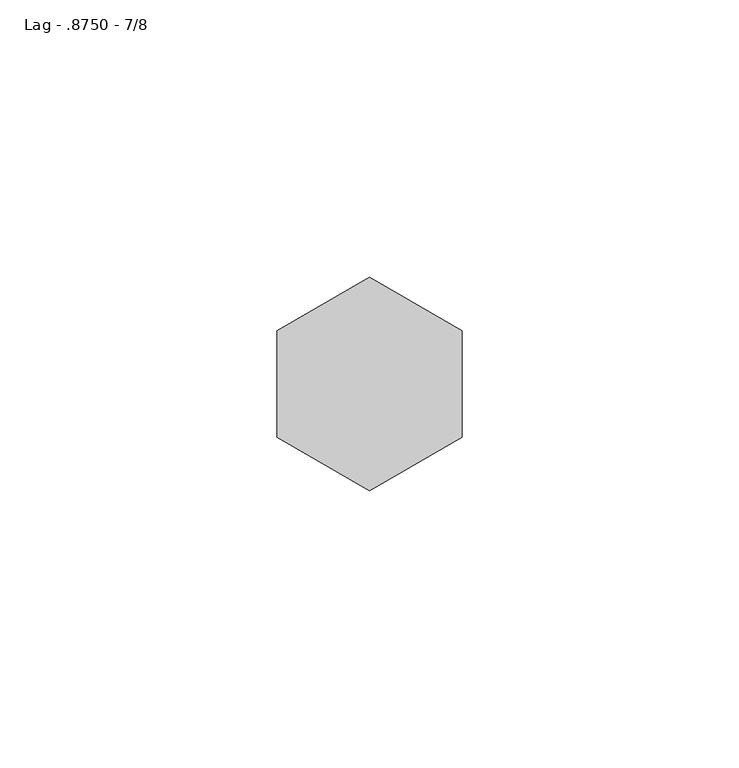
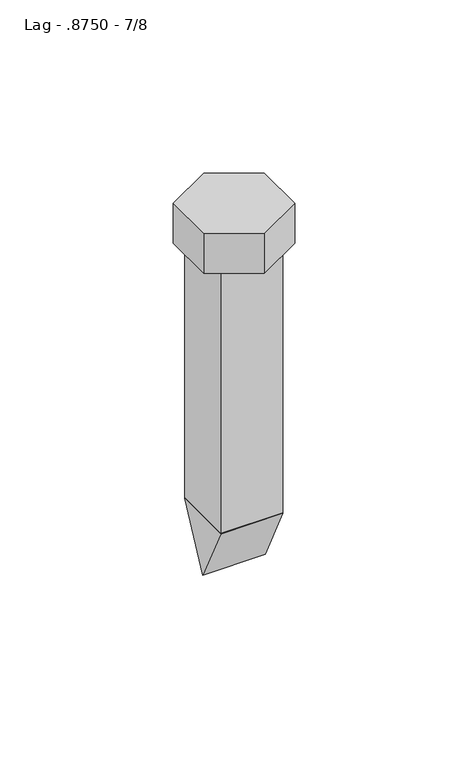
"""IFC4 building model written with IfcOpenShell, lengths in millimetres: fastener geometry, 060523 - W_P_C - Fastenings - Generic - SQUARE : Lag - .8750 - 7/8."""

from ifc_helpers import new_model, si_unit, frame, origin, origin_with_axes, place, context, project, spatial, polyline, outline, extrude, source, transform, mapped, element, save


def lag_8750_7_8_9ca2a517(model_context):
    return source(origin(), model_context, "Body", "SweptSolid", [
        extrude(outline(polyline([(0.0, -124.3210937), (-11.3605469, -101.6), (11.3605469, -101.6), (0.0, -124.3210937)])), frame((-11.3605469, 0.0, 0.0), z_axis=(1.0, 0.0, 0.0), x_axis=(0.0, 1.0, 0.0)), (0.0, 0.0, 1.0), 22.7210938),
        extrude(outline(polyline([(-16.66875, 9.6237073), (0.0, 19.2474146), (16.66875, 9.6237073), (16.66875, -9.6237073), (0.0, -19.2474146), (-16.66875, -9.6237073), (-16.66875, 9.6237073)])), origin_with_axes(), (0.0, 0.0, 1.0), 15.3789062),
        extrude(outline(polyline([(-11.3605469, 11.3605469), (11.3605469, 11.3605469), (11.3605469, -11.3605469), (-11.3605469, -11.3605469), (-11.3605469, 11.3605469)])), frame((0.0, 0.0, -101.6), z_axis=(0.0, 0.0, 1.0), x_axis=(1.0, 0.0, 0.0)), (0.0, 0.0, 1.0), 101.6),
    ])


if __name__ == "__main__":
    model = new_model("IFC4")
    model_context = context("Model", 3, world=origin())
    ifc_project = project(units=[si_unit("LENGTHUNIT", "METRE", prefix="MILLI")], contexts=[model_context])
    site = spatial("IfcSite", under=ifc_project)
    building = spatial("IfcBuilding", under=site)
    placement = place(None, origin())
    lag_8750_7_8_shape = lag_8750_7_8_9ca2a517(model_context)
    element("IfcFastener", 1, ObjectType="060523 - W_P_C - Fastenings - Generic - SQUARE : Lag - .8750 - 7/8", at=placement, inside=building, context=model_context, shape_type="MappedRepresentation", body=[
        mapped(lag_8750_7_8_shape, transform((0.0, 0.0, 0.0), x_axis=(1.0, 0.0, 0.0), y_axis=(0.0, 1.0, 0.0), z_axis=(0.0, 0.0, 1.0))),
    ])
    save(model, "model.ifc")

# Revit data of these elements
# Type "060523 - W_P_C - Fastenings - Generic - SQUARE : Lag - .8750 - 7/8"
#   Washer_Thickness = 0' - 0.20182"
#   Washer Radius = 0' - 1.05273"
#   Washer Offset - Head = 0' - 0"
#   Washer Offset = 0' - 0"
#   Thickness_of_Substrate [instance default] = 0' - 1"
#   Side = 0' - 0.75879"
#   Radius = 0' - 0.44727"
#   Length [instance default] = 0' - 4"
#   Head Size = 0' - 1 5/16"
#   Head Radius = 0' - 0 21/32"
#   Head Height = 0' - 0 155/256"
#   Double Diameter = 0' - 1 101/128"
#   Diameter = 0' - 0 229/256"
#   Default Elevation = 4' - 0"
#   Washer_Nut_Visibility = no
#   Washer_Head_Visibility = no
#   Round_Head_Visibility = no
#   Point Visibility = yes
#   Nut_Visibility = no
#   Hex_Head_Visiblilty = yes
#   Washer Material = none
#   Bolt Material (Size) = AT SILL - FASTENER AT 24" O.C.
# Element 1 (IfcFastener, "060523 - W_P_C - Fastenings - Generic - SQUARE : Lag - .8750 - 7/8")
#   Materials on its faces: "AT SILL - FASTENER AT 24\" O.C."
# Materials
#   "AT SILL - FASTENER AT 24\" O.C.": class "Generic", colour RGB 120 120 120, transparency 0, Cost = 0
